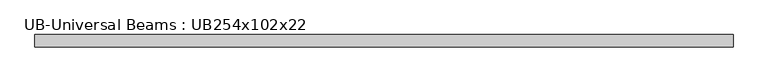
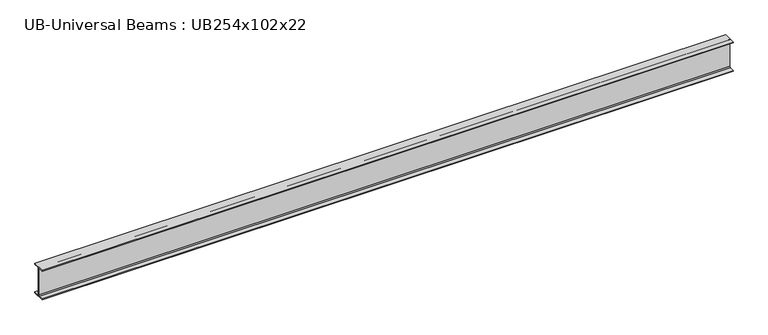
"""IFC4 building model written with IfcOpenShell, lengths in millimetres: beam geometry, UB-Universal Beams : UB254x102x22."""

from ifc_helpers import new_model, si_unit, point, frame, frame_2d, origin, place, context, project, spatial, polyline, circle_curve, trimmed, segment, composite_curve, outline, extrude, source, transform, mapped, element, save


def ub_universal_beams_ub254x102x22_fd37447c(model_context):
    return source(origin(), model_context, "Body", "SweptSolid", [
        extrude(outline(composite_curve([segment(polyline([(50.8, -120.2), (50.8, -127.0), (-50.8, -127.0), (-50.8, -120.2), (-10.45, -120.2)]), True, "CONTINUOUS"), segment(trimmed(circle_curve(frame_2d((-10.45, -112.6)), 7.6), [point((-10.45, -120.2))], [point((-2.85, -112.6))], True, "CARTESIAN"), True, "CONTINUOUS"), segment(polyline([(-2.85, -112.6), (-2.85, 112.6)]), True, "CONTINUOUS"), segment(trimmed(circle_curve(frame_2d((-10.45, 112.6)), 7.6), [point((-2.85, 112.6))], [point((-10.45, 120.2))], True, "CARTESIAN"), True, "CONTINUOUS"), segment(polyline([(-10.45, 120.2), (-50.8, 120.2), (-50.8, 127.0), (50.8, 127.0), (50.8, 120.2), (10.45, 120.2)]), True, "CONTINUOUS"), segment(trimmed(circle_curve(frame_2d((10.45, 112.6)), 7.6), [point((10.45, 120.2))], [point((2.85, 112.6))], True, "CARTESIAN"), True, "CONTINUOUS"), segment(polyline([(2.85, 112.6), (2.85, -112.6)]), True, "CONTINUOUS"), segment(trimmed(circle_curve(frame_2d((10.45, -112.6)), 7.6), [point((2.85, -112.6))], [point((10.45, -120.2))], True, "CARTESIAN"), True, "CONTINUOUS"), segment(polyline([(10.45, -120.2), (50.8, -120.2)]), True, "CONTINUOUS")], self_intersect=False)), frame((-2834.7, 0.0, 0.0), z_axis=(1.0, 0.0, 0.0), x_axis=(0.0, 1.0, 0.0)), (0.0, 0.0, 1.0), 5669.4),
    ])


if __name__ == "__main__":
    model = new_model("IFC4")
    model_context = context("Model", 3, world=origin())
    ifc_project = project(units=[si_unit("LENGTHUNIT", "METRE", prefix="MILLI")], contexts=[model_context])
    site = spatial("IfcSite", under=ifc_project)
    building = spatial("IfcBuilding", under=site)
    placement = place(None, origin())
    ub_universal_beams_ub254x102x22_shape = ub_universal_beams_ub254x102x22_fd37447c(model_context)
    element("IfcBeam", 1, ObjectType="UB-Universal Beams : UB254x102x22", at=placement, inside=building, context=model_context, shape_type="MappedRepresentation", body=[
        mapped(ub_universal_beams_ub254x102x22_shape, transform((0.0, 0.0, 0.0), x_axis=(1.0, 0.0, 0.0), y_axis=(0.0, 1.0, 0.0), z_axis=(0.0, 0.0, 1.0))),
    ])
    save(model, "model.ifc")

# Revit data of these elements
# Type "UB-Universal Beams : UB254x102x22"
#   Section Name Key = "UB254X102X22"
#   Width = 10.16 cm
#   Web Thickness = 0.57 cm
#   Web Fillet = 0.76 cm
#   Warping Constant = 18200.0 cm⁶
#   Torsional Moment of Inertia = 4.15 cm⁴
#   Section Area = 28.0 cm²
#   Plastic Modulus weak axis = 37.3 cm³
#   Plastic Modulus strong axis = 259.0 cm³
#   Nominal Weight = 22.00 kgf/m
#   Moment of Inertia weak axis = 119.00 cm⁴
#   Moment of Inertia strong axis = 2841.00 cm⁴
#   Height = 25.4 cm
#   Flange Thickness = 0.68 cm
#   Elastic Modulus weak axis = 23.5 cm³
#   Elastic Modulus strong axis = 224.0 cm³
#   Centroid Vertical = 12.7 cm
#   Centroid Horizontal = 5.08 cm
#   Bolt Spacing = 5.4 cm
#   Length [instance default] = 1500 mm
#   Structural Material [instance default] = Metal - Steel 43-275
#   Type Comments = ""
#   Assembly Code = ""
# Element 1 (IfcBeam, "UB-Universal Beams : UB254x102x22")
#   Materials on its faces: "Metal - Steel 43-275"
# Materials
#   "Metal - Steel 43-275": class "Metal", colour RGB 247 247 247, transparency 0, Cost = 0
